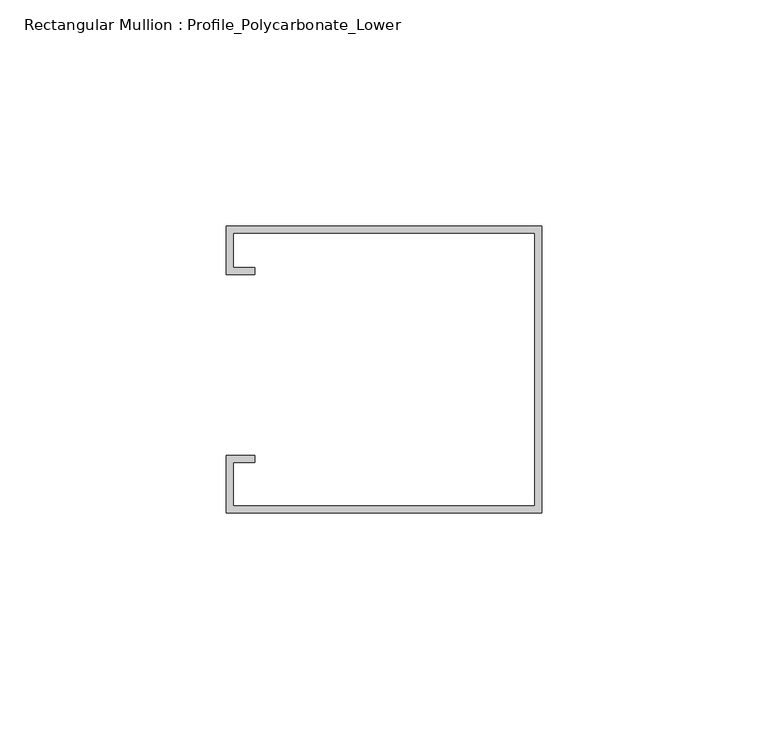
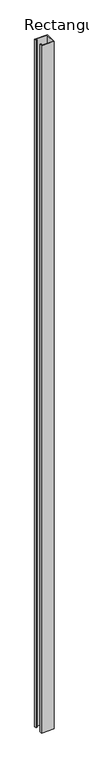
"""IFC4 building model written with IfcOpenShell, lengths in millimetres: member geometry, Rectangular Mullion : Profile_Polycarbonate_Lower."""

from ifc_helpers import new_model, si_unit, frame, origin, place, context, project, spatial, polyline, outline, extrude, source, transform, mapped, element, save


def rectangular_mullion_profile_polycarbonate_lower_487a61d3(model_context):
    return source(origin(), model_context, "Body", "SweptSolid", [
        extrude(outline(polyline([(0.0, -32.7), (-69.85, -32.7), (-69.85, -20.0), (-63.5, -20.0), (-63.5, -21.5875), (-68.2625, -21.5875), (-68.2625, -31.1125), (-1.5875, -31.1125), (-1.5875, 29.2125), (-68.2625, 29.2125), (-68.2625, 21.5875), (-63.5, 21.5875), (-63.5, 20.0), (-69.85, 20.0), (-69.85, 30.8), (0.0, 30.8), (0.0, -32.7)])), frame((0.0, 0.0, -4022.725), z_axis=(0.0, 0.0, 1.0), x_axis=(1.0, 0.0, 0.0)), (0.0, 0.0, 1.0), 4022.725),
    ])


if __name__ == "__main__":
    model = new_model("IFC4")
    model_context = context("Model", 3, world=origin())
    ifc_project = project(units=[si_unit("LENGTHUNIT", "METRE", prefix="MILLI")], contexts=[model_context])
    site = spatial("IfcSite", under=ifc_project)
    building = spatial("IfcBuilding", under=site)
    placement = place(None, origin())
    rectangular_mullion_profile_polycarbonate_lower_shape = rectangular_mullion_profile_polycarbonate_lower_487a61d3(model_context)
    element("IfcMember", 1, ObjectType="Rectangular Mullion : Profile_Polycarbonate_Lower", at=placement, inside=building, context=model_context, shape_type="MappedRepresentation", body=[
        mapped(rectangular_mullion_profile_polycarbonate_lower_shape, transform((0.0, 0.0, 0.0), x_axis=(1.0, 0.0, 0.0), y_axis=(0.0, 1.0, 0.0), z_axis=(0.0, 0.0, 1.0))),
    ])
    save(model, "model.ifc")

# Revit data of these elements
# Type "Rectangular Mullion : Profile_Polycarbonate_Lower"
#   built-in parameter 1007322 = 0.208333 (stored number, unit not read)
#   built-in parameter 1007321 = 0 (stored number, unit not read)
#   built-in parameter 1007320 = 0.00520833 (stored number, unit not read)
# Element 1 (IfcMember, "Rectangular Mullion : Profile_Polycarbonate_Lower")
#   Materials on its faces: "Aluminum"
# Materials
#   "Aluminum": class "Metal", colour RGB 244 244 244, transparency 0, Description = "Aluminum 6061", Cost = 0
